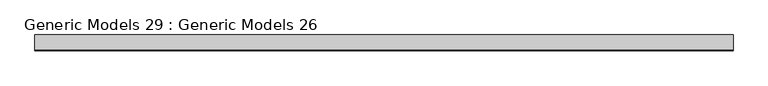
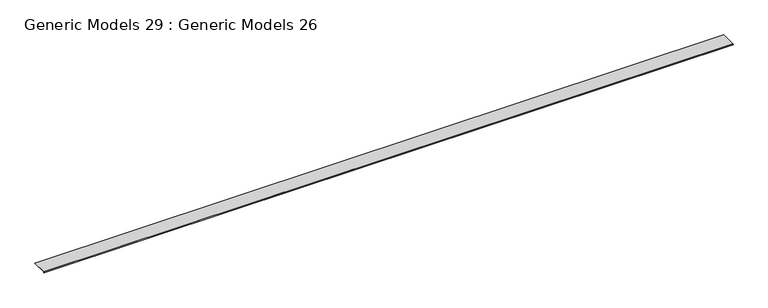
"""IFC4 building model written with IfcOpenShell, lengths in millimetres: proxy geometry, Generic Models 29 : Generic Models 26."""

from ifc_helpers import new_model, si_unit, frame, origin, place, context, project, spatial, polyline, outline, extrude, source, transform, mapped, element, save


def generic_models_29_generic_models_26_bf0ac949(model_context):
    return source(origin(), model_context, "Body", "SweptSolid", [
        extrude(outline(polyline([(25622.6249078, 266091.19375), (25490.0686578, 266091.19375), (25485.5785297, 266086.7036219), (25484.4559977, 266087.826154), (25489.4110937, 266092.78125), (25622.6249078, 266092.78125), (25622.6249078, 266091.19375)])), frame((27760.6090778, 0.0, 0.0), z_axis=(1.0, 0.0, 0.0), x_axis=(0.0, 1.0, 0.0)), (0.0, 0.0, 1.0), 6032.7256636),
    ])


if __name__ == "__main__":
    model = new_model("IFC4")
    model_context = context("Model", 3, world=origin())
    ifc_project = project(units=[si_unit("LENGTHUNIT", "METRE", prefix="MILLI")], contexts=[model_context])
    site = spatial("IfcSite", under=ifc_project)
    building = spatial("IfcBuilding", under=site)
    placement = place(None, origin())
    generic_models_29_generic_models_26_shape = generic_models_29_generic_models_26_bf0ac949(model_context)
    element("IfcBuildingElementProxy", 1, Name="Generic Models 29 : Generic Models 26", ObjectType="Generic Models 29 : Generic Models 26", at=placement, inside=building, context=model_context, shape_type="MappedRepresentation", body=[
        mapped(generic_models_29_generic_models_26_shape, transform((0.0, 0.0, 0.0), x_axis=(1.0, 0.0, 0.0), y_axis=(0.0, 1.0, 0.0), z_axis=(0.0, 0.0, 1.0))),
    ])
    save(model, "model.ifc")

# Revit data of these elements
# Element 1 (IfcBuildingElementProxy, "Generic Models 29 : Generic Models 26")
#   Materials on its faces: "GALV. BRAKE METAL - (COLOR: GALV.)"
# Materials
#   "GALV. BRAKE METAL - (COLOR: GALV.)": class "Generic", colour RGB 234 234 234, transparency 0, Cost = 0
